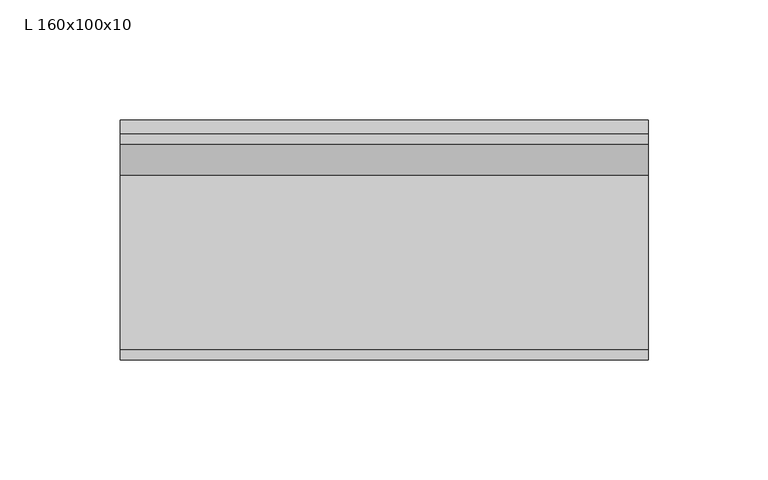
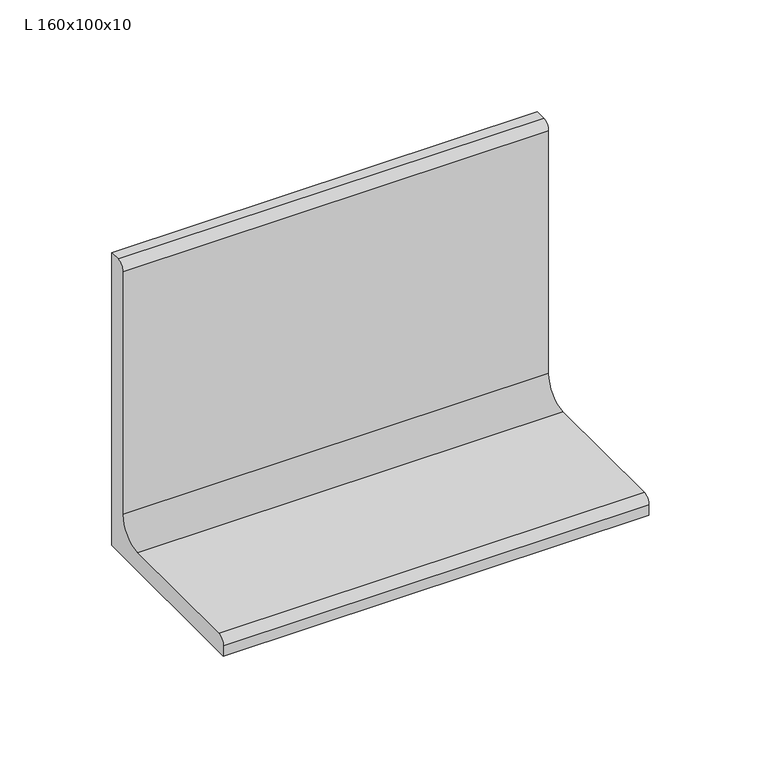
"""IFC4 building model written with IfcOpenShell, lengths in millimetres: beam geometry, Уголок (ГОСТ 8510-86) Балки : L 160x100x10."""

from ifc_helpers import new_model, si_unit, point, frame, frame_2d, origin, place, context, project, spatial, polyline, circle_curve, trimmed, segment, composite_curve, outline, extrude, source, transform, mapped, element, save


def l_160x100x10_a4cc4382(model_context):
    return source(origin(), model_context, "Body", "SweptSolid", [
        extrude(outline(composite_curve([segment(polyline([(22.8, -52.3), (-77.2, -52.3), (-77.2, -46.6)]), True, "CONTINUOUS"), segment(trimmed(circle_curve(frame_2d((-72.9, -46.6)), 4.3), [point((-77.2, -46.6))], [point((-72.9, -42.3))], False, "CARTESIAN"), True, "CONTINUOUS"), segment(polyline([(-72.9, -42.3), (-0.2, -42.3)]), True, "CONTINUOUS"), segment(trimmed(circle_curve(frame_2d((-0.2, -29.3)), 13.0), [point((-0.2, -42.3))], [point((12.8, -29.3))], True, "CARTESIAN"), True, "CONTINUOUS"), segment(polyline([(12.8, -29.3), (12.8, 103.4)]), True, "CONTINUOUS"), segment(trimmed(circle_curve(frame_2d((17.1, 103.4)), 4.3), [point((12.8, 103.4))], [point((17.1, 107.7))], False, "CARTESIAN"), True, "CONTINUOUS"), segment(polyline([(17.1, 107.7), (22.8, 107.7), (22.8, -52.3)]), True, "CONTINUOUS")], self_intersect=False)), frame((-110.0, 0.0, 0.0), z_axis=(1.0, 0.0, 0.0), x_axis=(0.0, 1.0, 0.0)), (0.0, 0.0, 1.0), 220.0),
    ])


if __name__ == "__main__":
    model = new_model("IFC4")
    model_context = context("Model", 3, world=origin())
    ifc_project = project(units=[si_unit("LENGTHUNIT", "METRE", prefix="MILLI")], contexts=[model_context])
    site = spatial("IfcSite", under=ifc_project)
    building = spatial("IfcBuilding", under=site)
    placement = place(None, origin())
    l_160x100x10_shape = l_160x100x10_a4cc4382(model_context)
    element("IfcBeam", 1, ObjectType="Уголок (ГОСТ 8510-86) Балки : L 160x100x10", at=placement, inside=building, context=model_context, shape_type="MappedRepresentation", body=[
        mapped(l_160x100x10_shape, transform((0.0, 0.0, 0.0), x_axis=(1.0, 0.0, 0.0), y_axis=(0.0, 1.0, 0.0), z_axis=(0.0, 0.0, 1.0))),
    ])
    save(model, "model.ifc")

# Revit data of these elements
# Type "Уголок (ГОСТ 8510-86) Балки : L 160x100x10"
#   ri = 4.3 mm
#   ra = 13 mm
#   W = 0.194662
#   Vz = 107.7 mm
#   Vy = 77.2 mm
#   Vpz = 52.3 mm
#   Vpy = 22.8 mm
#   Length [instance default] = 1500 mm
#   bf = 100 mm
#   d = 160 mm
#   tf = 10 mm
#   tw = 10 mm
#   A = 0.002528 m²
#   Structural Material [instance default] = Металл - Сталь - 345 МПa
#   Assembly Code = ""
# Element 1 (IfcBeam, "Уголок (ГОСТ 8510-86) Балки : L 160x100x10")
#   Structural Material = C235
#   Materials on its faces: "C235"
# Materials
#   "Металл - Сталь - 345 МПa": class "Металл", colour RGB 247 247 247, transparency 0
#   "C235": class "Не назначено", colour RGB 0 0 0, transparency 0
